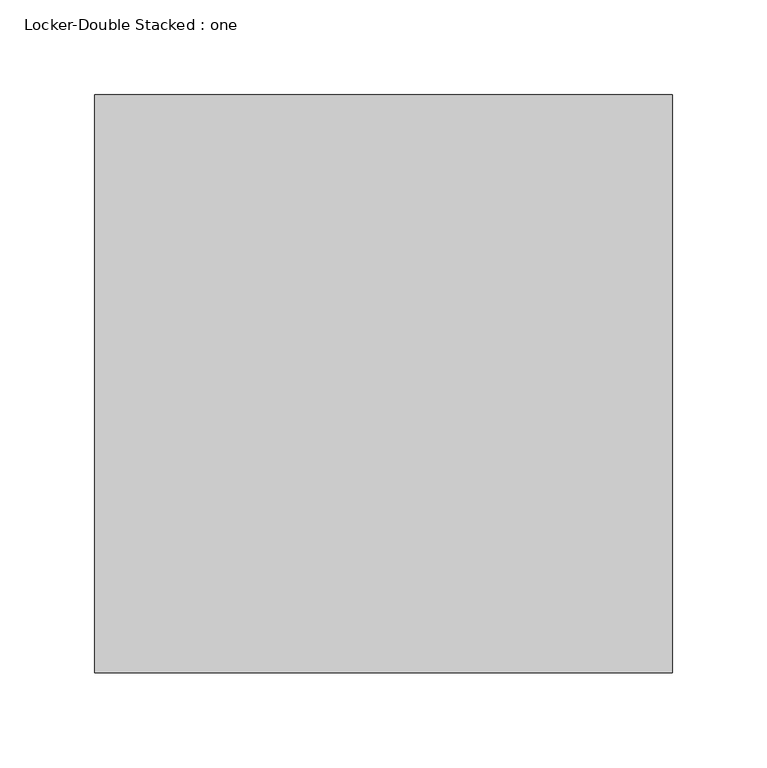
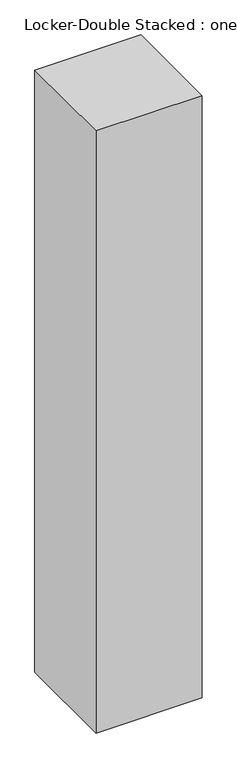
"""IFC4 building model written with IfcOpenShell, lengths in millimetres: furniture geometry, Locker-Double Stacked : one."""

from ifc_helpers import new_model, si_unit, origin, place, context, project, spatial, faceted_brep, source, transform, mapped, element, save


def locker_double_stacked_one_8e8d9ebb(model_context):
    return source(origin(), model_context, "Body", "Brep", [
        faceted_brep([(152.4, 152.4, 1828.8), (-152.4, 152.4, 1828.8), (-152.4, -152.4, 1828.8), (152.4, -152.4, 1828.8), (152.4, 152.4, 0.0), (152.4, -152.4, 0.0), (-152.4, -152.4, 0.0), (-152.4, 152.4, 0.0), (127.0, 152.4, 889.0), (-127.0, 152.4, 889.0), (-127.0, 152.4, 76.2), (127.0, 152.4, 76.2), (-127.0, 152.4, 1752.6), (-127.0, 152.4, 939.8), (127.0, 152.4, 939.8), (127.0, 152.4, 1752.6), (127.0, 146.05, 76.2), (-127.0, 146.05, 76.2), (-127.0, 146.05, 889.0), (127.0, 146.05, 889.0), (127.0, 146.05, 1752.6), (127.0, 146.05, 939.8), (-127.0, 146.05, 939.8), (-127.0, 146.05, 1752.6)], [[[0, 1, 2, 3]], [[4, 5, 6, 7]], [[3, 5, 4, 0]], [[2, 6, 5, 3]], [[1, 7, 6, 2]], [[0, 4, 7, 1], [8, 9, 10, 11], [12, 13, 14, 15]], [[16, 17, 18, 19]], [[19, 8, 11, 16]], [[18, 9, 8, 19]], [[17, 10, 9, 18]], [[16, 11, 10, 17]], [[20, 21, 22, 23]], [[23, 12, 15, 20]], [[22, 13, 12, 23]], [[21, 14, 13, 22]], [[20, 15, 14, 21]]]),
    ])


if __name__ == "__main__":
    model = new_model("IFC4")
    model_context = context("Model", 3, world=origin())
    ifc_project = project(units=[si_unit("LENGTHUNIT", "METRE", prefix="MILLI")], contexts=[model_context])
    site = spatial("IfcSite", under=ifc_project)
    building = spatial("IfcBuilding", under=site)
    placement = place(None, origin())
    locker_double_stacked_one_shape = locker_double_stacked_one_8e8d9ebb(model_context)
    element("IfcFurniture", 1, ObjectType="Locker-Double Stacked : one", at=placement, inside=building, context=model_context, shape_type="MappedRepresentation", body=[
        mapped(locker_double_stacked_one_shape, transform((0.0, 0.0, 0.0), x_axis=(1.0, 0.0, 0.0), y_axis=(0.0, 1.0, 0.0), z_axis=(0.0, 0.0, 1.0))),
    ])
    save(model, "model.ifc")

# Revit data of these elements
# Type "Locker-Double Stacked : one"
#   Keynote = "M10511300.01"
#   Keynote = "M10511300.01"
#   Assembly Code = "E2010"
#   Depth = 1' - 0"
#   Height = 6' - 0"
#   Width = 1' - 0"
#   Material = LOCKERS
# Element 1 (IfcFurniture, "Locker-Double Stacked : one")
#   Materials on its faces: "LOCKERS"
# Materials
#   "LOCKERS": class "Unassigned", colour RGB 98 98 98, transparency 0, Description = "Metal Painted", Cost = 0
